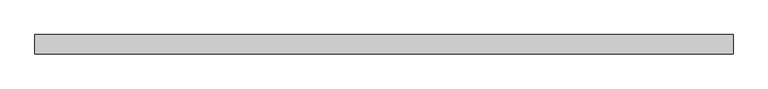
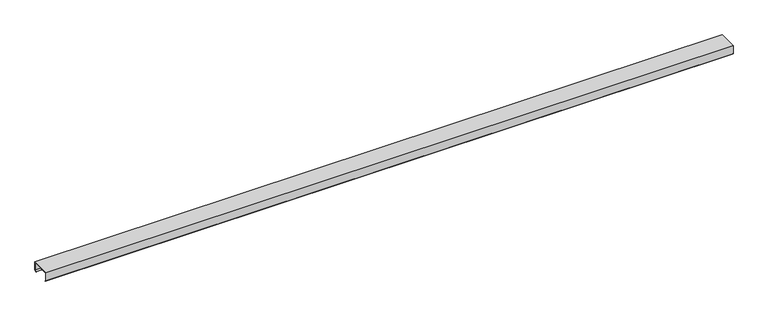
"""IFC4 building model written with IfcOpenShell, lengths in millimetres: proxy geometry, Generic Models 7:Generic Models 1:1:Generic Models 1:1 : Generic Models 7:Generic Models 1:337419:8 : Generic Models 7:Generic Models 1:1:Generic Models 1:1 : Generic Models 7:Generic Models 1:337419:306201."""

from ifc_helpers import new_model, si_unit, frame, origin, place, context, project, spatial, polyline, outline, extrude, source, transform, mapped, element, save


def generic_models_5b39e394(model_context):
    return source(origin(), model_context, "Body", "SweptSolid", [
        extrude(outline(polyline([(-579000.6913841, 4985.940625), (-578797.4913841, 4985.940625), (-578797.4913841, 4897.040625), (-578812.0845307, 4884.7955211), (-578813.8702751, 4886.9236883), (-578800.2695091, 4898.336086), (-578800.2695091, 4983.1625), (-578997.9132591, 4983.1625), (-578997.9132591, 4898.336086), (-578984.3124931, 4886.9236883), (-578986.0982375, 4884.7955211), (-579000.6913841, 4897.040625), (-579000.6913841, 4985.940625)])), frame((565582.1867239, 0.0, 0.0), z_axis=(1.0, 0.0, 0.0), x_axis=(0.0, 1.0, 0.0)), (0.0, 0.0, 1.0), 7315.2),
    ])


if __name__ == "__main__":
    model = new_model("IFC4")
    model_context = context("Model", 3, world=origin())
    ifc_project = project(units=[si_unit("LENGTHUNIT", "METRE", prefix="MILLI")], contexts=[model_context])
    site = spatial("IfcSite", under=ifc_project)
    building = spatial("IfcBuilding", under=site)
    placement = place(None, origin())
    generic_models_shape = generic_models_5b39e394(model_context)
    element("IfcBuildingElementProxy", 1, Name="Generic Models 7:Generic Models 1:1:Generic Models 1:1 : Generic Models 7:Generic Models 1:337419:8 : Generic Models 7:Generic Models 1:1:Generic Models 1:1 : Generic Models 7:Generic Models 1:337419:306201", ObjectType="Generic Models 7:Generic Models 1:1:Generic Models 1:1 : Generic Models 7:Generic Models 1:337419:8 : Generic Models 7:Generic Models 1:1:Generic Models 1:1 : Generic Models 7:Generic Models 1:337419:306201", at=placement, inside=building, context=model_context, shape_type="MappedRepresentation", body=[
        mapped(generic_models_shape, transform((0.0, 0.0, 0.0), x_axis=(1.0, 0.0, 0.0), y_axis=(0.0, 1.0, 0.0), z_axis=(0.0, 0.0, 1.0))),
    ])
    save(model, "model.ifc")

# Revit data of these elements
# Type "Generic Models 7:Generic Models 1:1:Generic Models 1:1 : Generic Models 7:Generic Models 1:337419:8 : Generic Models 7:Generic Models 1:1:Generic Models 1:1 : Generic Models 7:Generic Models 1:337419:306201"
#   NameOverride = "Generic Models 7:Generic Models 1:1:Generic Models 1:1 : Generic Models 7:Generic Models 1:337419:306201"
#   ObjectTypeOverride = "Generic Models 1:1 : Generic Models 7:Generic Models 1:337419"
#   Reference = "Generic Models 1"
#   Tag = "306201"
# Element 1 (IfcBuildingElementProxy, "Generic Models 7:Generic Models 1:1:Generic Models 1:1 : Generic Models 7:Generic Models 1:337419:8 : Generic Models 7:Generic Models 1:1:Generic Models 1:1 : Generic Models 7:Generic Models 1:337419:306201")
#   Materials on its faces: "CEE' SECTION (8.0x3.5C - SEE STRUCT. DWGS)"
# Materials
#   "CEE' SECTION (8.0x3.5C - SEE STRUCT. DWGS)": class "Unassigned", colour RGB 210 209 208, transparency 0, Keynote = "M05121300.02", Cost = 0
